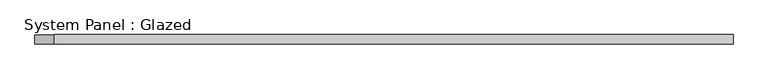
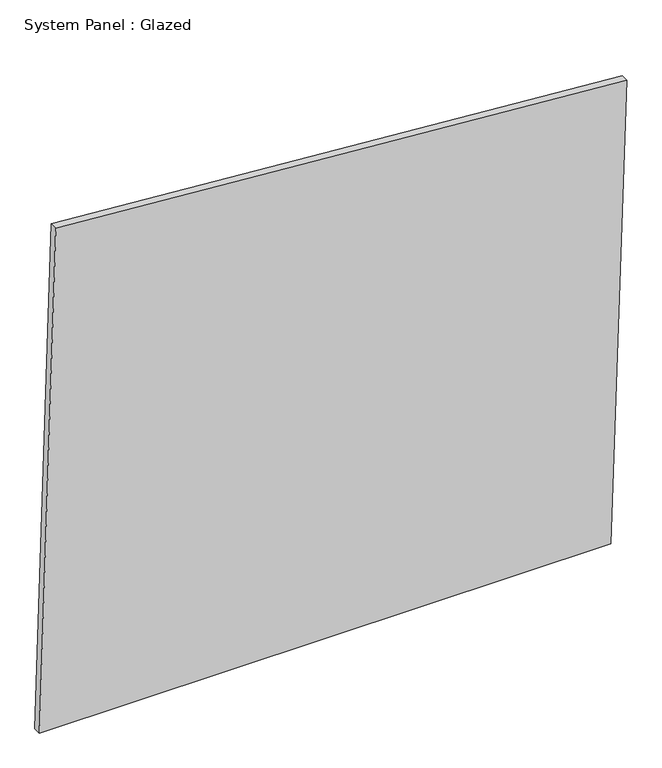
"""IFC4 building model written with IfcOpenShell, lengths in millimetres: plate geometry, System Panel : Glazed."""

from ifc_helpers import new_model, si_unit, frame, origin, place, context, project, spatial, polyline, outline, extrude, source, transform, mapped, element, save


def system_panel_glazed_08f6996d(model_context):
    return source(origin(), model_context, "Body", "SweptSolid", [
        extrude(outline(polyline([(0.0, -938.7563704), (0.0, 887.9536467), (1548.6739711, 938.7563704), (1687.2330704, -886.4668133), (0.0, -938.7563704)])), frame((0.0, -49.5, 0.0), z_axis=(0.0, 1.0, 0.0), x_axis=(0.0, 0.0, 1.0)), (0.0, 0.0, 1.0), 25.0),
    ])


if __name__ == "__main__":
    model = new_model("IFC4")
    model_context = context("Model", 3, world=origin())
    ifc_project = project(units=[si_unit("LENGTHUNIT", "METRE", prefix="MILLI")], contexts=[model_context])
    site = spatial("IfcSite", under=ifc_project)
    building = spatial("IfcBuilding", under=site)
    placement = place(None, origin())
    system_panel_glazed_shape = system_panel_glazed_08f6996d(model_context)
    element("IfcPlate", 1, ObjectType="System Panel : Glazed", at=placement, inside=building, context=model_context, shape_type="MappedRepresentation", body=[
        mapped(system_panel_glazed_shape, transform((0.0, 0.0, 0.0), x_axis=(1.0, 0.0, 0.0), y_axis=(0.0, 1.0, 0.0), z_axis=(0.0, 0.0, 1.0))),
    ])
    save(model, "model.ifc")

# Revit data of these elements
# Element 1 (IfcPlate, "System Panel : Glazed")
#   Materials on its faces: "Glass, Clear Glazing"
# Materials
#   "Glass, Clear Glazing": class "Glass", colour RGB 247 249 248, transparency 0.85, Description = "Clear glazing", Cost = 0
